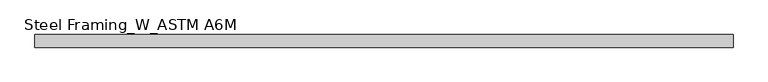
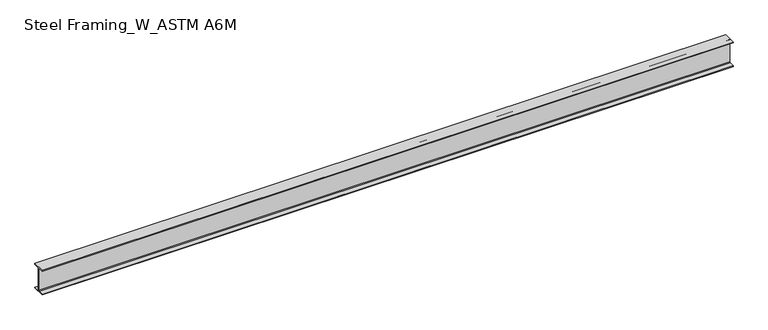
"""IFC4 building model written with IfcOpenShell, lengths in millimetres: beam geometry, Steel Framing_W_ASTM A6M : H_SB_AR_S02_W360x51_B4."""

from ifc_helpers import new_model, si_unit, point, frame, frame_2d, origin, place, context, project, spatial, polyline, circle_curve, trimmed, segment, composite_curve, outline, extrude, source, transform, mapped, element, save


def steel_framing_w_astm_a6m_0a603e5e(model_context):
    return source(origin(), model_context, "Body", "SweptSolid", [
        extrude(outline(composite_curve([segment(polyline([(85.5, -166.4), (85.5, -178.0), (-85.5, -178.0), (-85.5, -166.4), (-13.72, -166.4)]), True, "CONTINUOUS"), segment(trimmed(circle_curve(frame_2d((-13.72, -156.3)), 10.1), [point((-13.72, -166.4))], [point((-3.62, -156.3))], True, "CARTESIAN"), True, "CONTINUOUS"), segment(polyline([(-3.62, -156.3), (-3.62, 156.3)]), True, "CONTINUOUS"), segment(trimmed(circle_curve(frame_2d((-13.72, 156.3)), 10.1), [point((-3.62, 156.3))], [point((-13.72, 166.4))], True, "CARTESIAN"), True, "CONTINUOUS"), segment(polyline([(-13.72, 166.4), (-85.5, 166.4), (-85.5, 178.0), (85.5, 178.0), (85.5, 166.4), (13.72, 166.4)]), True, "CONTINUOUS"), segment(trimmed(circle_curve(frame_2d((13.72, 156.3)), 10.1), [point((13.72, 166.4))], [point((3.62, 156.3))], True, "CARTESIAN"), True, "CONTINUOUS"), segment(polyline([(3.62, 156.3), (3.62, -156.3)]), True, "CONTINUOUS"), segment(trimmed(circle_curve(frame_2d((13.72, -156.3)), 10.1), [point((3.62, -156.3))], [point((13.72, -166.4))], True, "CARTESIAN"), True, "CONTINUOUS"), segment(polyline([(13.72, -166.4), (85.5, -166.4)]), True, "CONTINUOUS")], self_intersect=False)), frame((-4717.9, 0.0, 0.0), z_axis=(1.0, 0.0, 0.0), x_axis=(0.0, 1.0, 0.0)), (0.0, 0.0, 1.0), 9464.7),
    ])


if __name__ == "__main__":
    model = new_model("IFC4")
    model_context = context("Model", 3, world=origin())
    ifc_project = project(units=[si_unit("LENGTHUNIT", "METRE", prefix="MILLI")], contexts=[model_context])
    site = spatial("IfcSite", under=ifc_project)
    building = spatial("IfcBuilding", under=site)
    placement = place(None, origin())
    steel_framing_w_astm_a6m_shape = steel_framing_w_astm_a6m_0a603e5e(model_context)
    element("IfcBeam", 1, ObjectType="Steel Framing_W_ASTM A6M : H_SB_AR_S02_W360x51_B4", at=placement, inside=building, context=model_context, shape_type="MappedRepresentation", body=[
        mapped(steel_framing_w_astm_a6m_shape, transform((0.0, 0.0, 0.0), x_axis=(1.0, 0.0, 0.0), y_axis=(0.0, 1.0, 0.0), z_axis=(0.0, 0.0, 1.0))),
    ])
    save(model, "model.ifc")

# Revit data of these elements
# Type "Steel Framing_W_ASTM A6M : H_SB_AR_S02_W360x51_B4"
#   Type Mark = "B4"
#   Section Name Key = "W14x34"
#   Width = 17.1 cm
#   Web Thickness = 0.724 cm
#   Web Fillet = 1.01 cm
#   Warping Constant = 287000.0 cm⁶
#   Torsional Moment of Inertia = 23.70 cm⁴
#   Section Area = 64.5 cm²
#   Plastic Modulus weak axis = 174.0 cm³
#   Plastic Modulus strong axis = 895.0 cm³
#   Perimeter = 1.36 m²/m
#   Nominal Weight = 51.00 kgf/m
#   Moment of Inertia weak axis = 970.00 cm⁴
#   Moment of Inertia strong axis = 14200.00 cm⁴
#   Height = 35.6 cm
#   Flange Thickness = 1.16 cm
#   Elastic Modulus weak axis = 113.0 cm³
#   Elastic Modulus strong axis = 796.0 cm³
#   Centroid Vertical = 17.8 cm
#   Centroid Horizontal = 8.55 cm
#   Length [instance default] = 1500 mm
#   Structural Material [instance default] = Steel, 45-345
#   Bolt Spacing = 0
#   Assembly Code = ""
# Element 1 (IfcBeam, "Steel Framing_W_ASTM A6M : H_SB_AR_S02_W360x51_B4")
#   Materials on its faces: "Steel, 45-345"
# Materials
#   "Steel, 45-345": class "Metal", colour RGB 189 187 185, transparency 0, Description = "Steel 345 MPa", Cost = 0
